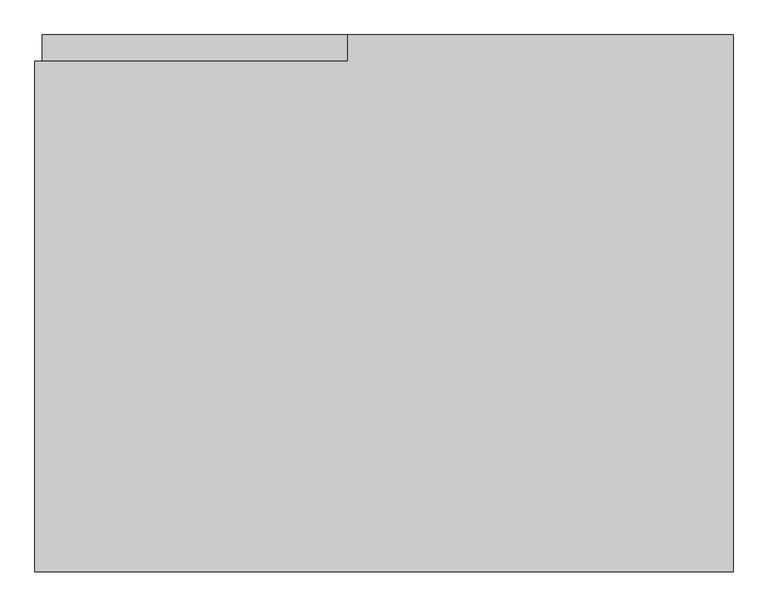
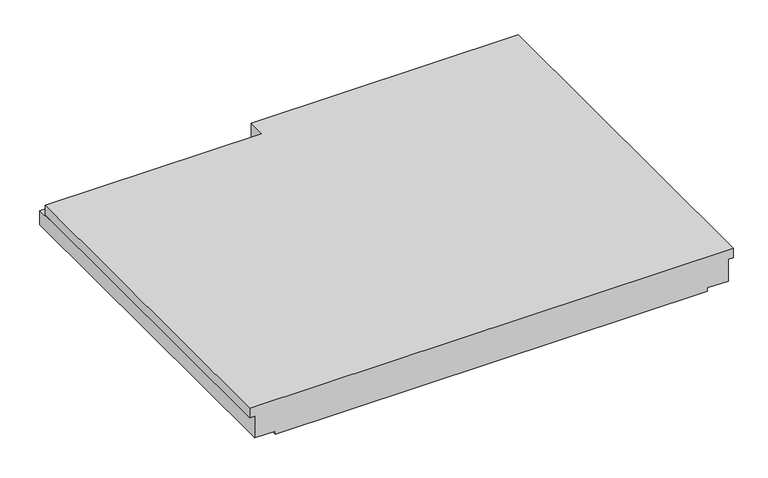
"""IFC4 building model written with IfcOpenShell, lengths in millimetres: stair geometry, NLRS_24_GM_UN_rechthoekig bordes prefab zonder oplegnok-AV_gen_rsf : prefab bordes_gen__2250x2925."""

from ifc_helpers import new_model, si_unit, origin, place, context, project, spatial, faceted_brep, source, transform, mapped, element, save


def stair_1f2f9ad8(model_context):
    return source(origin(), model_context, "Body", "Brep", [
        faceted_brep([(1462.5, 2250.0, 0.0), (1462.5, 0.0, 0.0), (1462.5, 0.0, -60.0), (1462.5, 2250.0, -60.0), (-152.5, 2250.0, 0.0), (-152.5, 2250.0, -110.0), (-152.5, 2140.0, -110.0), (-152.5, 2140.0, 0.0), (-1462.5, 0.0, 0.0), (-1462.5, 2140.0, 0.0), (-1462.5, 2140.0, -60.0), (-1462.5, 0.0, -60.0), (-1432.5, 2250.0, -110.0), (1432.5, 2250.0, -60.0), (1432.5, 2250.0, -200.0), (1307.5, 2250.0, -200.0), (1307.5, 2250.0, -220.0), (-1307.5, 2250.0, -220.0), (-1307.5, 2250.0, -200.0), (-1432.5, 2250.0, -200.0), (-1432.5, 2140.0, -110.0), (-1432.5, 2140.0, -60.0), (-1432.5, 0.0, -60.0), (-1432.5, 0.0, -200.0), (-1307.5, 0.0, -200.0), (-1307.5, 0.0, -220.0), (1307.5, 0.0, -220.0), (1307.5, 0.0, -200.0), (1432.5, 0.0, -200.0), (1432.5, 0.0, -60.0)], [[[0, 1, 2, 3]], [[4, 5, 6, 7]], [[8, 9, 10, 11]], [[12, 5, 4, 0, 3, 13, 14, 15, 16, 17, 18, 19]], [[5, 12, 20, 6]], [[9, 7, 6, 20, 21, 10]], [[9, 8, 1, 0, 4, 7]], [[8, 11, 22, 23, 24, 25, 26, 27, 28, 29, 2, 1]], [[25, 17, 16, 26]], [[21, 22, 11, 10]], [[19, 23, 22, 21, 20, 12]], [[23, 19, 18, 24]], [[24, 18, 17, 25]], [[29, 13, 3, 2]], [[13, 29, 28, 14]], [[14, 28, 27, 15]], [[15, 27, 26, 16]]]),
    ])


if __name__ == "__main__":
    model = new_model("IFC4")
    model_context = context("Model", 3, world=origin())
    ifc_project = project(units=[si_unit("LENGTHUNIT", "METRE", prefix="MILLI")], contexts=[model_context])
    site = spatial("IfcSite", under=ifc_project)
    building = spatial("IfcBuilding", under=site)
    placement = place(None, origin())
    stair_shape = stair_1f2f9ad8(model_context)
    element("IfcStair", 1, ObjectType="NLRS_24_GM_UN_rechthoekig bordes prefab zonder oplegnok-AV_gen_rsf : prefab bordes_gen__2250x2925", at=placement, inside=building, context=model_context, shape_type="MappedRepresentation", body=[
        mapped(stair_shape, transform((0.0, 0.0, 0.0), x_axis=(1.0, 0.0, 0.0), y_axis=(0.0, 1.0, 0.0), z_axis=(0.0, 0.0, 1.0))),
    ])
    save(model, "model.ifc")

# Revit data of these elements
# Type "NLRS_24_GM_UN_rechthoekig bordes prefab zonder oplegnok-AV_gen_rsf : prefab bordes_gen__2250x2925"
#   IfcExportAs = "IfcStair"
#   Type Comments = " "
#   Model = " "
#   Manufacturer = " "
#   Description = "rechthoekig bordes prefab\r\n1930x4395"
#   Assembly Code = "24.15"
#   Width = 2925 mm
#   Thickness = 220 mm
#   Perimeter = 10350 mm
#   NLRS_C_lengte_02 = 1310 mm
#   NLRS_C_lengte_01 = 1310 mm
#   NLRS_C_hoogte_02 = 110 mm
#   NLRS_C_hoogte_01 = 110 mm
#   NLRS_C_diepte_04 = 2250 mm
#   NLRS_C_diepte_03 = 2250 mm
#   NLRS_C_diepte_02 = 110 mm
#   NLRS_C_diepte_01 = 110 mm
#   Length = 2250 mm
#   Default Elevation = 1219.2 mm
#   Area = 6.58125 m²
#   NLRS_C_materiaal = NLRS_f2_beton prefab_gen_rsf
#   Keynote = ""
# Element 1 (IfcStair, "NLRS_24_GM_UN_rechthoekig bordes prefab zonder oplegnok-AV_gen_rsf : prefab bordes_gen__2250x2925")
#   Materials on its faces: "NLRS_f2_beton prefab_gen_rsf"
# Materials
#   "NLRS_f2_beton prefab_gen_rsf": class "F - Niet gebakken kunststeen", colour RGB 129 133 118, transparency 0, Keynote = "f2", Manufacturer = "Revit Standards Foundation", URL = "www.revitstandards.org", Description = "beton prefab", Cost = 0
